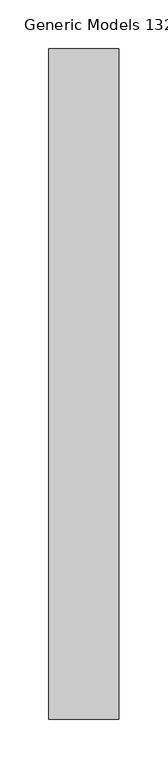
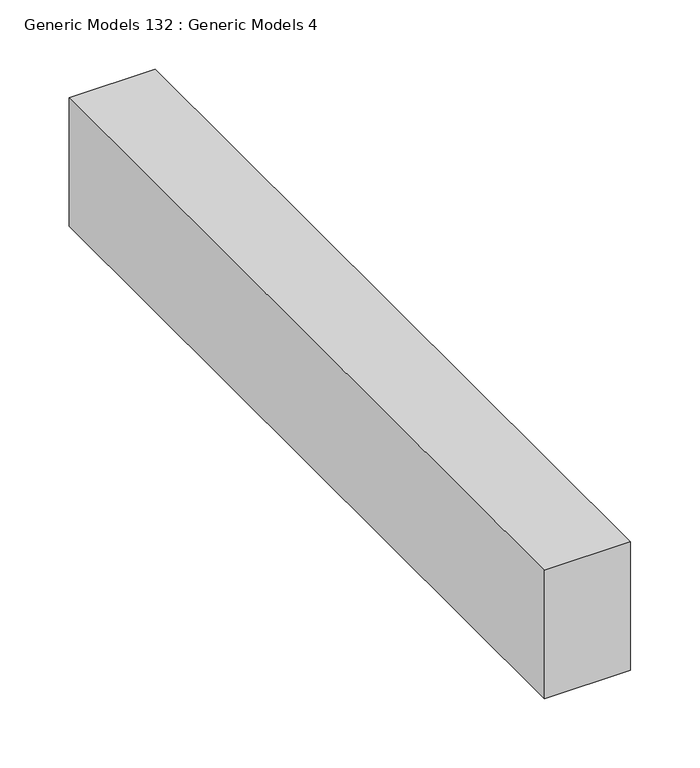
"""IFC4 building model written with IfcOpenShell, lengths in millimetres: proxy geometry, Generic Models 132 : Generic Models 4."""

from ifc_helpers import new_model, si_unit, frame, origin, place, context, project, spatial, polyline, outline, extrude, source, transform, mapped, element, save


def generic_models_132_generic_models_4_679f8ecb(model_context):
    return source(origin(), model_context, "Body", "SweptSolid", [
        extrude(outline(polyline([(-318.6717702, 1085.2769662), (-247.1350514, 1085.2769662), (-247.1350514, 399.7309662), (-318.6717702, 399.7309662), (-318.6717702, 1085.2769662)])), frame((0.0, 0.0, 126359.2889687), z_axis=(0.0, 0.0, 1.0), x_axis=(1.0, 0.0, 0.0)), (0.0, 0.0, 1.0), 113.109375),
    ])


if __name__ == "__main__":
    model = new_model("IFC4")
    model_context = context("Model", 3, world=origin())
    ifc_project = project(units=[si_unit("LENGTHUNIT", "METRE", prefix="MILLI")], contexts=[model_context])
    site = spatial("IfcSite", under=ifc_project)
    building = spatial("IfcBuilding", under=site)
    placement = place(None, origin())
    generic_models_132_generic_models_4_shape = generic_models_132_generic_models_4_679f8ecb(model_context)
    element("IfcBuildingElementProxy", 1, Name="Generic Models 132 : Generic Models 4", ObjectType="Generic Models 132 : Generic Models 4", at=placement, inside=building, context=model_context, shape_type="MappedRepresentation", body=[
        mapped(generic_models_132_generic_models_4_shape, transform((0.0, 0.0, 0.0), x_axis=(1.0, 0.0, 0.0), y_axis=(0.0, 1.0, 0.0), z_axis=(0.0, 0.0, 1.0))),
    ])
    save(model, "model.ifc")

# Revit data of these elements
# Element 1 (IfcBuildingElementProxy, "Generic Models 132 : Generic Models 4")
#   Materials on its faces: "_BLOCKING AS REQUIRED"
# Materials
#   "_BLOCKING AS REQUIRED": class "Generic", colour RGB 177 130 114, transparency 0, Cost = 0
